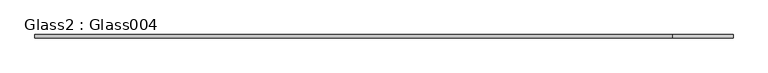
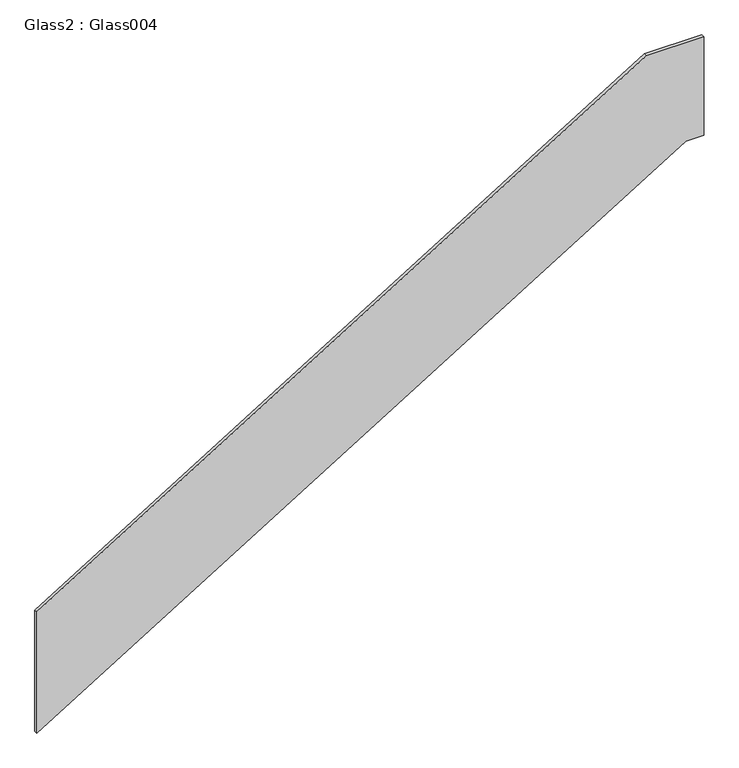
"""IFC4 building model written with IfcOpenShell, lengths in millimetres: proxy geometry, Glass2 : Glass004."""

import ifcopenshell
import ifcopenshell.guid

model = None  # the IFC model being written
_history = None  # IfcOwnerHistory: only IFC2X3 demands one
_inside = {}  # id of a spatial element -> (the spatial element, [elements in it])
_under = {}  # id of a project, library or spatial element -> (it, [spatial elements below it])
_declared = {}  # id of a project -> (the project, [libraries it declares])
_typed = {}  # id of a type object -> (the type object, [elements of that type])
_made_of = {}  # id of a material, layer set ... -> (it, [elements and type objects made of it])


def new_model(schema):
    """Start an empty IFC model of exactly this schema.

    Asked for "IFC4X3", IfcOpenShell would pick the latest addendum, in which some entities
    have other attributes; the version numbers below select the first issue.
    IFC2X3 requires an IfcOwnerHistory on every rooted entity: one is made here for all.
    """
    global model, _history
    if schema == "IFC4X3":
        model = ifcopenshell.file(schema_version=(4, 3, 0, 0))
    else:
        model = ifcopenshell.file(schema=schema)
    _inside.clear()
    _under.clear()
    _declared.clear()
    _typed.clear()
    _made_of.clear()
    _history = None
    if model.schema == "IFC2X3":
        org = make("IfcOrganization", Name="unknown")
        user = make(
            "IfcPersonAndOrganization",
            ThePerson=make("IfcPerson", FamilyName="unknown"),
            TheOrganization=org,
        )
        app = make(
            "IfcApplication",
            ApplicationDeveloper=org,
            Version="unknown",
            ApplicationFullName="unknown",
            ApplicationIdentifier="unknown",
        )
        _history = make(
            "IfcOwnerHistory",
            OwningUser=user,
            OwningApplication=app,
            ChangeAction="ADDED",
            CreationDate=0,
        )
    return model


def make(cls, **values):
    """One entity of the class cls with the attributes given. An attribute that is None is left unset."""
    return model.create_entity(
        cls, **{name: value for name, value in values.items() if value is not None}
    )


def rooted(cls, **values):
    """An entity with a GlobalId (a new one), such as an element, a storey or a relation."""
    return make(cls, GlobalId=ifcopenshell.guid.new(), OwnerHistory=_history, **values)


def si_unit(unit_type, name, prefix=None):
    """IfcSIUnit, for example si_unit("LENGTHUNIT", "METRE", prefix="MILLI")."""
    return make("IfcSIUnit", UnitType=unit_type, Prefix=prefix, Name=name)


def assignment(units):
    """IfcUnitAssignment: the units of a project."""
    return None if units is None else make("IfcUnitAssignment", Units=units)


def point(xyz):
    """IfcCartesianPoint."""
    return None if xyz is None else make("IfcCartesianPoint", Coordinates=xyz)


def direction(xyz):
    """IfcDirection."""
    return None if xyz is None else make("IfcDirection", DirectionRatios=xyz)


def frame(location, z_axis=None, x_axis=None):
    """IfcAxis2Placement3D, a coordinate frame: its origin and axes. An axis left out is left unset."""
    return make(
        "IfcAxis2Placement3D",
        Location=point(location),
        Axis=direction(z_axis),
        RefDirection=direction(x_axis),
    )


def origin():
    """The frame at (0, 0, 0) with its axes left unset."""
    return frame((0.0, 0.0, 0.0))


def place(relative_to, where):
    """IfcLocalPlacement: puts the frame where relative to a parent placement (None: the world)."""
    return make(
        "IfcLocalPlacement", PlacementRelTo=relative_to, RelativePlacement=where
    )


def context(
    kind, dimensions, precision=None, world=None, true_north=None, identifier=None
):
    """IfcGeometricRepresentationContext, for example the 3D "Model" context."""
    return make(
        "IfcGeometricRepresentationContext",
        ContextIdentifier=identifier,
        ContextType=kind,
        CoordinateSpaceDimension=dimensions,
        Precision=precision,
        WorldCoordinateSystem=world,
        TrueNorth=true_north,
    )


def project(units=None, contexts=None):
    """IfcProject with its units and contexts."""
    return rooted(
        "IfcProject",
        Name="project",
        RepresentationContexts=contexts,
        UnitsInContext=assignment(units),
    )


def spatial(cls, under=None, at=None, **own):
    """A site, building, storey or space (cls), placed at a placement, below another one or the project."""
    s = rooted(cls, ObjectPlacement=at, **own)
    if under is not None:
        _under.setdefault(under.id(), (under, []))[1].append(s)
    return s


def polyline(points):
    """IfcPolyline through the points."""
    return make("IfcPolyline", Points=[point(p) for p in points])


def outline(outer, holes=None, kind="AREA"):
    """IfcArbitraryClosedProfileDef: a profile drawn as a closed curve; with holes, ...WithVoids."""
    if holes is None:
        return make("IfcArbitraryClosedProfileDef", ProfileType=kind, OuterCurve=outer)
    return make(
        "IfcArbitraryProfileDefWithVoids",
        ProfileType=kind,
        OuterCurve=outer,
        InnerCurves=holes,
    )


def extrude(swept, where, along, depth):
    """IfcExtrudedAreaSolid: the profile swept, set in the frame where, extruded along a direction by depth."""
    return make(
        "IfcExtrudedAreaSolid",
        SweptArea=swept,
        Position=where,
        ExtrudedDirection=direction(along),
        Depth=depth,
    )


def shape(context_of_items, identifier, shape_type, items):
    """IfcShapeRepresentation: the items that make up one representation, for example the "Body"."""
    return make(
        "IfcShapeRepresentation",
        ContextOfItems=context_of_items,
        RepresentationIdentifier=identifier,
        RepresentationType=shape_type,
        Items=items,
    )


def source(mapping_origin, context_of_items, identifier, shape_type, items):
    """IfcRepresentationMap: a shape defined once, which mapped items show again and again."""
    return make(
        "IfcRepresentationMap",
        MappingOrigin=mapping_origin,
        MappedRepresentation=shape(context_of_items, identifier, shape_type, items),
    )


def transform(
    local_origin,
    x_axis=None,
    y_axis=None,
    z_axis=None,
    scale=None,
    scale2=None,
    scale3=None,
    uniform=True,
):
    """IfcCartesianTransformationOperator3D, or its non-uniform kind. x_axis, y_axis, z_axis: its Axis1, 2, 3."""
    if uniform:
        return make(
            "IfcCartesianTransformationOperator3D",
            Axis1=direction(x_axis),
            Axis2=direction(y_axis),
            LocalOrigin=point(local_origin),
            Scale=scale,
            Axis3=direction(z_axis),
        )
    return make(
        "IfcCartesianTransformationOperator3DnonUniform",
        Axis1=direction(x_axis),
        Axis2=direction(y_axis),
        LocalOrigin=point(local_origin),
        Scale=scale,
        Axis3=direction(z_axis),
        Scale2=scale2,
        Scale3=scale3,
    )


def mapped(mapping_source, mapping_target):
    """IfcMappedItem: shows the shape of a source again, moved by a transform."""
    return make(
        "IfcMappedItem", MappingSource=mapping_source, MappingTarget=mapping_target
    )


def made_of(thing, what):
    """Note that an element or type object is made of a material, layer set ...; save() writes the relation."""
    if what is not None:
        _made_of.setdefault(what.id(), (what, []))[1].append(thing)
    return thing


def element(
    cls,
    number,
    at=None,
    inside=None,
    cuts=None,
    type_object=None,
    material=None,
    context=None,
    identifier="Body",
    shape_type=None,
    held_by="IfcProductDefinitionShape",
    body=None,
    shapes=None,
    **own,
):
    """One element of the class cls, such as IfcWall. Its Tag is "e" and its number.

    at: its placement. inside: the storey or other place that contains it. cuts: it is an
    opening in that element (IfcRelVoidsElement). A single representation is given by context,
    identifier, shape_type and body (its items); several are given by shapes. held_by: the class
    of the entity that holds the representations. save() writes the other relations.
    """
    e = rooted(cls, Tag="e%d" % number, ObjectPlacement=at, **own)
    if body is not None:
        shapes = [shape(context, identifier, shape_type, body)]
    if shapes is not None:
        e.Representation = make(held_by, Representations=shapes)
    if inside is not None:
        _inside.setdefault(inside.id(), (inside, []))[1].append(e)
    if cuts is not None:
        rooted(
            "IfcRelVoidsElement", RelatingBuildingElement=cuts, RelatedOpeningElement=e
        )
    if type_object is not None:
        _typed.setdefault(type_object.id(), (type_object, []))[1].append(e)
    return made_of(e, material)


def aggregate(whole, parts):
    """IfcRelAggregates: a whole, such as a stair, and the parts it consists of."""
    return rooted("IfcRelAggregates", RelatingObject=whole, RelatedObjects=parts)


def save(model, path):
    """Write the relations noted so far, then the file.

    IfcRelAggregates (storeys below a building ...), IfcRelContainedInSpatialStructure (elements
    in a storey), IfcRelDefinesByType, IfcRelAssociatesMaterial and IfcRelDeclares: one each for
    every whole, place, type object, material and project.
    """
    for whole, parts in _under.values():
        aggregate(whole, parts)
    for where, things in _inside.values():
        rooted(
            "IfcRelContainedInSpatialStructure",
            RelatedElements=things,
            RelatingStructure=where,
        )
    for kind, things in _typed.values():
        rooted("IfcRelDefinesByType", RelatedObjects=things, RelatingType=kind)
    for what, things in _made_of.values():
        rooted("IfcRelAssociatesMaterial", RelatedObjects=things, RelatingMaterial=what)
    for by, libraries in _declared.values():
        rooted("IfcRelDeclares", RelatingContext=by, RelatedDefinitions=libraries)
    model.write(path)


def glass2_glass004_a8b2c382(model_context):
    return source(origin(), model_context, "Body", "SweptSolid", [
        extrude(outline(polyline([(38035.9266566, 4990.3637308), (37022.6954344, 4990.3637308), (40173.1410997, 10124.4233335), (40173.1410997, 10267.8101348), (40995.0266566, 10267.8101348), (40995.0266566, 9812.6007679), (38035.9266566, 4990.3637308)])), frame((0.0, 888.7781447, 0.0), z_axis=(0.0, 1.0, 0.0), x_axis=(0.0, 0.0, 1.0)), (0.0, 0.0, 1.0), 25.6840222),
    ])


if __name__ == "__main__":
    model = new_model("IFC4")
    model_context = context("Model", 3, world=origin())
    ifc_project = project(units=[si_unit("LENGTHUNIT", "METRE", prefix="MILLI")], contexts=[model_context])
    site = spatial("IfcSite", under=ifc_project)
    building = spatial("IfcBuilding", under=site)
    placement = place(None, origin())
    glass2_glass004_shape = glass2_glass004_a8b2c382(model_context)
    element("IfcBuildingElementProxy", 1, Name="Glass2 : Glass004", ObjectType="Glass2 : Glass004", at=placement, inside=building, context=model_context, shape_type="MappedRepresentation", body=[
        mapped(glass2_glass004_shape, transform((0.0, 0.0, 0.0), x_axis=(1.0, 0.0, 0.0), y_axis=(0.0, 1.0, 0.0), z_axis=(0.0, 0.0, 1.0))),
    ])
    save(model, "model.ifc")

# Revit data of these elements
# Type "Glass2 : Glass004"
#   NameOverride = "Glass004"
# Element 1 (IfcBuildingElementProxy, "Glass2 : Glass004")
#   Materials on its faces: "1/2\" TEMPERED GLASS"
# Materials
#   "1/2\" TEMPERED GLASS": class "Unassigned", colour RGB 191 240 251, transparency 0, Cost = 0
